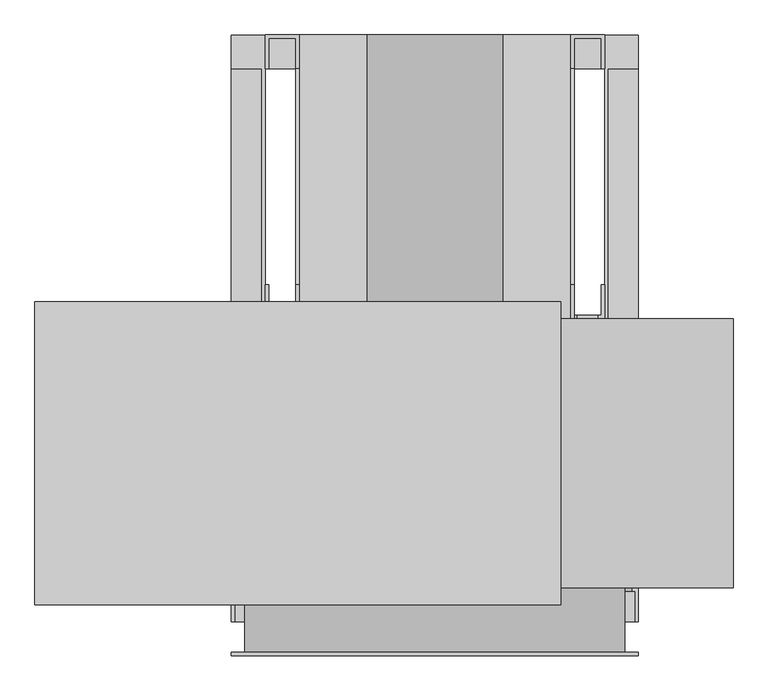
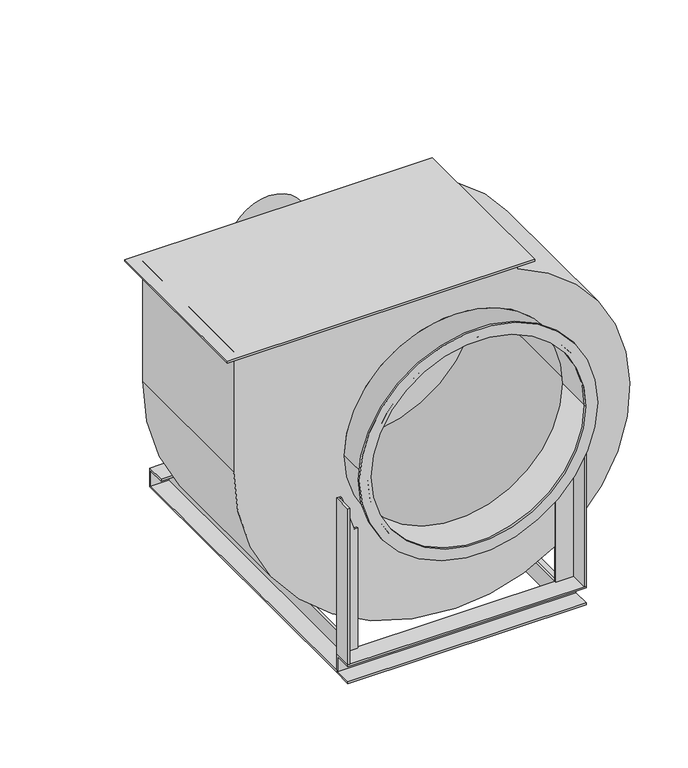
"""IFC4 building model written with IfcOpenShell, lengths in millimetres: proxy geometry, ВЕЗА_Вентилятор ВРАН : ВРАН6-056."""

import ifcopenshell
import ifcopenshell.guid

model = None  # the IFC model being written
_history = None  # IfcOwnerHistory: only IFC2X3 demands one
_inside = {}  # id of a spatial element -> (the spatial element, [elements in it])
_under = {}  # id of a project, library or spatial element -> (it, [spatial elements below it])
_declared = {}  # id of a project -> (the project, [libraries it declares])
_typed = {}  # id of a type object -> (the type object, [elements of that type])
_made_of = {}  # id of a material, layer set ... -> (it, [elements and type objects made of it])


def new_model(schema):
    """Start an empty IFC model of exactly this schema.

    Asked for "IFC4X3", IfcOpenShell would pick the latest addendum, in which some entities
    have other attributes; the version numbers below select the first issue.
    IFC2X3 requires an IfcOwnerHistory on every rooted entity: one is made here for all.
    """
    global model, _history
    if schema == "IFC4X3":
        model = ifcopenshell.file(schema_version=(4, 3, 0, 0))
    else:
        model = ifcopenshell.file(schema=schema)
    _inside.clear()
    _under.clear()
    _declared.clear()
    _typed.clear()
    _made_of.clear()
    _history = None
    if model.schema == "IFC2X3":
        org = make("IfcOrganization", Name="unknown")
        user = make(
            "IfcPersonAndOrganization",
            ThePerson=make("IfcPerson", FamilyName="unknown"),
            TheOrganization=org,
        )
        app = make(
            "IfcApplication",
            ApplicationDeveloper=org,
            Version="unknown",
            ApplicationFullName="unknown",
            ApplicationIdentifier="unknown",
        )
        _history = make(
            "IfcOwnerHistory",
            OwningUser=user,
            OwningApplication=app,
            ChangeAction="ADDED",
            CreationDate=0,
        )
    return model


def make(cls, **values):
    """One entity of the class cls with the attributes given. An attribute that is None is left unset."""
    return model.create_entity(
        cls, **{name: value for name, value in values.items() if value is not None}
    )


def rooted(cls, **values):
    """An entity with a GlobalId (a new one), such as an element, a storey or a relation."""
    return make(cls, GlobalId=ifcopenshell.guid.new(), OwnerHistory=_history, **values)


def si_unit(unit_type, name, prefix=None):
    """IfcSIUnit, for example si_unit("LENGTHUNIT", "METRE", prefix="MILLI")."""
    return make("IfcSIUnit", UnitType=unit_type, Prefix=prefix, Name=name)


def assignment(units):
    """IfcUnitAssignment: the units of a project."""
    return None if units is None else make("IfcUnitAssignment", Units=units)


def point(xyz):
    """IfcCartesianPoint."""
    return None if xyz is None else make("IfcCartesianPoint", Coordinates=xyz)


def direction(xyz):
    """IfcDirection."""
    return None if xyz is None else make("IfcDirection", DirectionRatios=xyz)


def frame(location, z_axis=None, x_axis=None):
    """IfcAxis2Placement3D, a coordinate frame: its origin and axes. An axis left out is left unset."""
    return make(
        "IfcAxis2Placement3D",
        Location=point(location),
        Axis=direction(z_axis),
        RefDirection=direction(x_axis),
    )


def frame_2d(location, x_axis=None):
    """IfcAxis2Placement2D, a coordinate frame in the plane: its origin and x axis."""
    return make(
        "IfcAxis2Placement2D", Location=point(location), RefDirection=direction(x_axis)
    )


def origin():
    """The frame at (0, 0, 0) with its axes left unset."""
    return frame((0.0, 0.0, 0.0))


def place(relative_to, where):
    """IfcLocalPlacement: puts the frame where relative to a parent placement (None: the world)."""
    return make(
        "IfcLocalPlacement", PlacementRelTo=relative_to, RelativePlacement=where
    )


def context(
    kind, dimensions, precision=None, world=None, true_north=None, identifier=None
):
    """IfcGeometricRepresentationContext, for example the 3D "Model" context."""
    return make(
        "IfcGeometricRepresentationContext",
        ContextIdentifier=identifier,
        ContextType=kind,
        CoordinateSpaceDimension=dimensions,
        Precision=precision,
        WorldCoordinateSystem=world,
        TrueNorth=true_north,
    )


def project(units=None, contexts=None):
    """IfcProject with its units and contexts."""
    return rooted(
        "IfcProject",
        Name="project",
        RepresentationContexts=contexts,
        UnitsInContext=assignment(units),
    )


def spatial(cls, under=None, at=None, **own):
    """A site, building, storey or space (cls), placed at a placement, below another one or the project."""
    s = rooted(cls, ObjectPlacement=at, **own)
    if under is not None:
        _under.setdefault(under.id(), (under, []))[1].append(s)
    return s


def polyline(points):
    """IfcPolyline through the points."""
    return make("IfcPolyline", Points=[point(p) for p in points])


def circle_curve(where, radius):
    """IfcCircle in the frame where."""
    return make("IfcCircle", Position=where, Radius=radius)


def trimmed(basis, trim1, trim2, sense, master):
    """IfcTrimmedCurve: the piece of a basis curve between two trims."""
    return make(
        "IfcTrimmedCurve",
        BasisCurve=basis,
        Trim1=trim1,
        Trim2=trim2,
        SenseAgreement=sense,
        MasterRepresentation=master,
    )


def segment(curve, same_sense, transition):
    """IfcCompositeCurveSegment."""
    return make(
        "IfcCompositeCurveSegment",
        Transition=transition,
        SameSense=same_sense,
        ParentCurve=curve,
    )


def composite_curve(segments, self_intersect=None):
    """IfcCompositeCurve: segments joined end to end."""
    return make("IfcCompositeCurve", Segments=segments, SelfIntersect=self_intersect)


def outline(outer, holes=None, kind="AREA"):
    """IfcArbitraryClosedProfileDef: a profile drawn as a closed curve; with holes, ...WithVoids."""
    if holes is None:
        return make("IfcArbitraryClosedProfileDef", ProfileType=kind, OuterCurve=outer)
    return make(
        "IfcArbitraryProfileDefWithVoids",
        ProfileType=kind,
        OuterCurve=outer,
        InnerCurves=holes,
    )


def extrude(swept, where, along, depth):
    """IfcExtrudedAreaSolid: the profile swept, set in the frame where, extruded along a direction by depth."""
    return make(
        "IfcExtrudedAreaSolid",
        SweptArea=swept,
        Position=where,
        ExtrudedDirection=direction(along),
        Depth=depth,
    )


def faces_of(points, faces, orient=None, outer=None):
    """IfcFace entities. A face is a list of loops; a loop is a list of indices into points, from 0.

    orient and outer hold one flag for each loop. By default every Orientation is true, the
    first loop of a face is its IfcFaceOuterBound and the others are IfcFaceBound.
    """
    made = []
    for i, loops in enumerate(faces):
        bounds = []
        for j, loop in enumerate(loops):
            is_outer = j == 0 if outer is None else outer[i][j]
            bounds.append(
                make(
                    "IfcFaceOuterBound" if is_outer else "IfcFaceBound",
                    Bound=make("IfcPolyLoop", Polygon=[points[k] for k in loop]),
                    Orientation=True if orient is None else orient[i][j],
                )
            )
        made.append(make("IfcFace", Bounds=bounds))
    return made


def faceted_brep(points, faces, orient=None, outer=None, voids=None):
    """IfcFacetedBrep: a solid bounded by flat faces; with voids (closed shells), ...WithVoids."""
    shared = [point(p) for p in points]
    hull = make("IfcClosedShell", CfsFaces=faces_of(shared, faces, orient, outer))
    if voids is None:
        return make("IfcFacetedBrep", Outer=hull)
    return make(
        "IfcFacetedBrepWithVoids",
        Outer=hull,
        Voids=[
            make(cls, CfsFaces=faces_of(shared, fs, o, b)) for cls, fs, o, b in voids
        ],
    )


def shape(context_of_items, identifier, shape_type, items):
    """IfcShapeRepresentation: the items that make up one representation, for example the "Body"."""
    return make(
        "IfcShapeRepresentation",
        ContextOfItems=context_of_items,
        RepresentationIdentifier=identifier,
        RepresentationType=shape_type,
        Items=items,
    )


def source(mapping_origin, context_of_items, identifier, shape_type, items):
    """IfcRepresentationMap: a shape defined once, which mapped items show again and again."""
    return make(
        "IfcRepresentationMap",
        MappingOrigin=mapping_origin,
        MappedRepresentation=shape(context_of_items, identifier, shape_type, items),
    )


def transform(
    local_origin,
    x_axis=None,
    y_axis=None,
    z_axis=None,
    scale=None,
    scale2=None,
    scale3=None,
    uniform=True,
):
    """IfcCartesianTransformationOperator3D, or its non-uniform kind. x_axis, y_axis, z_axis: its Axis1, 2, 3."""
    if uniform:
        return make(
            "IfcCartesianTransformationOperator3D",
            Axis1=direction(x_axis),
            Axis2=direction(y_axis),
            LocalOrigin=point(local_origin),
            Scale=scale,
            Axis3=direction(z_axis),
        )
    return make(
        "IfcCartesianTransformationOperator3DnonUniform",
        Axis1=direction(x_axis),
        Axis2=direction(y_axis),
        LocalOrigin=point(local_origin),
        Scale=scale,
        Axis3=direction(z_axis),
        Scale2=scale2,
        Scale3=scale3,
    )


def mapped(mapping_source, mapping_target):
    """IfcMappedItem: shows the shape of a source again, moved by a transform."""
    return make(
        "IfcMappedItem", MappingSource=mapping_source, MappingTarget=mapping_target
    )


def made_of(thing, what):
    """Note that an element or type object is made of a material, layer set ...; save() writes the relation."""
    if what is not None:
        _made_of.setdefault(what.id(), (what, []))[1].append(thing)
    return thing


def element(
    cls,
    number,
    at=None,
    inside=None,
    cuts=None,
    type_object=None,
    material=None,
    context=None,
    identifier="Body",
    shape_type=None,
    held_by="IfcProductDefinitionShape",
    body=None,
    shapes=None,
    **own,
):
    """One element of the class cls, such as IfcWall. Its Tag is "e" and its number.

    at: its placement. inside: the storey or other place that contains it. cuts: it is an
    opening in that element (IfcRelVoidsElement). A single representation is given by context,
    identifier, shape_type and body (its items); several are given by shapes. held_by: the class
    of the entity that holds the representations. save() writes the other relations.
    """
    e = rooted(cls, Tag="e%d" % number, ObjectPlacement=at, **own)
    if body is not None:
        shapes = [shape(context, identifier, shape_type, body)]
    if shapes is not None:
        e.Representation = make(held_by, Representations=shapes)
    if inside is not None:
        _inside.setdefault(inside.id(), (inside, []))[1].append(e)
    if cuts is not None:
        rooted(
            "IfcRelVoidsElement", RelatingBuildingElement=cuts, RelatedOpeningElement=e
        )
    if type_object is not None:
        _typed.setdefault(type_object.id(), (type_object, []))[1].append(e)
    return made_of(e, material)


def aggregate(whole, parts):
    """IfcRelAggregates: a whole, such as a stair, and the parts it consists of."""
    return rooted("IfcRelAggregates", RelatingObject=whole, RelatedObjects=parts)


def save(model, path):
    """Write the relations noted so far, then the file.

    IfcRelAggregates (storeys below a building ...), IfcRelContainedInSpatialStructure (elements
    in a storey), IfcRelDefinesByType, IfcRelAssociatesMaterial and IfcRelDeclares: one each for
    every whole, place, type object, material and project.
    """
    for whole, parts in _under.values():
        aggregate(whole, parts)
    for where, things in _inside.values():
        rooted(
            "IfcRelContainedInSpatialStructure",
            RelatedElements=things,
            RelatingStructure=where,
        )
    for kind, things in _typed.values():
        rooted("IfcRelDefinesByType", RelatedObjects=things, RelatingType=kind)
    for what, things in _made_of.values():
        rooted("IfcRelAssociatesMaterial", RelatedObjects=things, RelatingMaterial=what)
    for by, libraries in _declared.values():
        rooted("IfcRelDeclares", RelatingContext=by, RelatedDefinitions=libraries)
    model.write(path)


def mechanical_equipment_89e30f27(model_context):
    return source(origin(), model_context, "Body", "SolidModel", [
        extrude(outline(polyline([(185.5, 223.5), (185.5, -223.5), (-589.5, -223.5), (-589.5, 223.5), (185.5, 223.5)])), frame((0.0, 0.0, 940.0), z_axis=(0.0, 0.0, 1.0), x_axis=(1.0, 0.0, 0.0)), (0.0, 0.0, 1.0), 5.0),
        extrude(outline(composite_curve([segment(trimmed(circle_curve(frame_2d((625.0, 0.5002234)), 560.0002234), [point((625.0, -559.5))], [point((65.0, 0.0))], False, "CARTESIAN"), True, "CONTINUOUS"), segment(trimmed(circle_curve(frame_2d((504.1653304, 0.3189338)), 439.1654462), [point((65.0, 0.0))], [point((915.0, 155.5))], False, "CARTESIAN"), True, "CONTINUOUS"), segment(polyline([(915.0, 155.5), (945.0, 155.5), (945.0, -559.5), (625.0, -559.5)]), True, "CONTINUOUS")], self_intersect=False), holes=[composite_curve([segment(trimmed(circle_curve(frame_2d((570.0, 0.0)), 280.0), [point((570.0, -280.0))], [point((570.0, 280.0))], True, "CARTESIAN"), True, "CONTINUOUS"), segment(trimmed(circle_curve(frame_2d((570.0, 0.0)), 280.0), [point((570.0, 280.0))], [point((570.0, -280.0))], True, "CARTESIAN"), True, "CONTINUOUS")], self_intersect=False)]), frame((0.0, -198.5, 0.0), z_axis=(0.0, 1.0, 0.0), x_axis=(0.0, 0.0, 1.0)), (0.0, 0.0, 1.0), 397.0),
        faceted_brep([(-300.0, 611.5, 5.0), (-300.0, 611.5, 45.0), (-300.0, 566.5, 45.0), (-300.0, 566.5, 50.0), (-300.0, 616.5, 50.0), (-300.0, 616.5, 0.0), (-300.0, -198.5, 0.0), (-300.0, -198.5, 5.0), (300.0, 616.5, 50.0), (300.0, 566.5, 50.0), (300.0, 566.5, 45.0), (300.0, 611.5, 45.0), (300.0, 611.5, 5.0), (300.0, -198.5, 5.0), (300.0, -198.5, 0.0), (300.0, 616.5, 0.0), (250.0, -198.5, 0.0), (250.0, 566.5, 0.0), (-250.0, 566.5, 0.0), (-250.0, -198.5, 0.0), (-255.0, 566.5, 45.0), (-255.0, 566.5, 50.0), (255.0, 566.5, 50.0), (255.0, 566.5, 45.0), (-200.0, 566.5, 470.0), (-205.0, 566.5, 470.0), (-205.0, 566.5, 50.0), (-245.0, 566.5, 50.0), (-245.0, 566.5, 470.0), (-250.0, 566.5, 470.0), (-250.0, 566.5, 50.0), (250.0, 566.5, 50.0), (250.0, 566.5, 470.0), (245.0, 566.5, 470.0), (245.0, 566.5, 50.0), (205.0, 566.5, 50.0), (205.0, 566.5, 470.0), (200.0, 566.5, 470.0), (200.0, 566.5, 50.0), (-200.0, 566.5, 50.0), (205.0, 566.5, 5.0), (205.0, 566.5, 45.0), (245.0, 566.5, 45.0), (245.0, 566.5, 5.0), (-245.0, 566.5, 5.0), (-245.0, 566.5, 45.0), (-205.0, 566.5, 45.0), (-205.0, 566.5, 5.0), (-200.0, 566.5, 5.0), (-200.0, 566.5, 45.0), (200.0, 566.5, 45.0), (200.0, 566.5, 5.0), (245.0, 611.5, 5.0), (205.0, 611.5, 5.0), (-205.0, 611.5, 5.0), (-245.0, 611.5, 5.0), (200.0, 611.5, 5.0), (-200.0, 611.5, 5.0), (255.0, -198.5, 5.0), (255.0, 611.5, 5.0), (-255.0, -198.5, 5.0), (-255.0, 611.5, 5.0), (-255.0, 611.5, 45.0), (255.0, 611.5, 45.0), (245.0, 611.5, 45.0), (205.0, 611.5, 45.0), (-205.0, 611.5, 45.0), (-245.0, 611.5, 45.0), (200.0, 611.5, 45.0), (-200.0, 611.5, 45.0), (-255.0, -198.5, 50.0), (-250.0, -198.5, 50.0), (-250.0, 616.5, 50.0), (250.0, 616.5, 50.0), (250.0, -198.5, 50.0), (255.0, -198.5, 50.0), (-205.0, 611.5, 50.0), (-245.0, 611.5, 50.0), (245.0, 611.5, 50.0), (205.0, 611.5, 50.0), (200.0, 616.5, 50.0), (-200.0, 616.5, 50.0), (-250.0, 616.5, 470.0), (-200.0, 616.5, 470.0), (200.0, 616.5, 470.0), (250.0, 616.5, 470.0), (-245.0, 611.5, 470.0), (-205.0, 611.5, 470.0), (205.0, 611.5, 470.0), (245.0, 611.5, 470.0)], [[[0, 1, 2, 3, 4, 5, 6, 7]], [[8, 9, 10, 11, 12, 13, 14, 15]], [[14, 16, 17, 18, 19, 6, 5, 15]], [[3, 2, 20, 21]], [[10, 9, 22, 23]], [[24, 25, 26, 27, 28, 29, 30, 18, 17, 31, 32, 33, 34, 35, 36, 37, 38, 39], [40, 41, 42, 43], [44, 45, 46, 47], [48, 49, 50, 51]], [[40, 43, 52, 53]], [[44, 47, 54, 55]], [[48, 51, 56, 57]], [[58, 13, 12, 59]], [[7, 60, 61, 0]], [[1, 0, 61, 62]], [[12, 11, 63, 59]], [[53, 52, 64, 65]], [[55, 54, 66, 67]], [[57, 56, 68, 69]], [[2, 1, 62, 20]], [[11, 10, 23, 63]], [[65, 64, 42, 41]], [[67, 66, 46, 45]], [[69, 68, 50, 49]], [[4, 3, 21, 70, 71, 30, 72]], [[9, 8, 73, 31, 74, 75, 22]], [[27, 26, 76, 77]], [[35, 34, 78, 79]], [[39, 38, 80, 81]], [[8, 15, 5, 4, 72, 82, 83, 81, 80, 84, 85, 73]], [[75, 74, 16, 14, 13, 58]], [[75, 58, 59, 63, 23, 22]], [[16, 74, 31, 17]], [[70, 60, 7, 6, 19, 71]], [[60, 70, 21, 20, 62, 61]], [[71, 19, 18, 30]], [[83, 82, 29, 28, 86, 87, 25, 24]], [[84, 37, 36, 88, 89, 33, 32, 85]], [[89, 88, 79, 78]], [[43, 42, 64, 52]], [[33, 89, 78, 34]], [[85, 32, 31, 73]], [[51, 50, 68, 56]], [[37, 84, 80, 38]], [[41, 40, 53, 65]], [[88, 36, 35, 79]], [[29, 82, 72, 30]], [[45, 44, 55, 67]], [[86, 28, 27, 77]], [[87, 86, 77, 76]], [[47, 46, 66, 54]], [[25, 87, 76, 26]], [[49, 48, 57, 69]], [[83, 24, 39, 81]]]),
        extrude(outline(polyline([(566.5, 0.0), (198.5, 0.0), (198.5, 770.0), (248.5420316, 770.0), (566.5, 510.0420316), (566.5, 0.0)]), holes=[polyline([(248.5, 495.0), (486.5, 495.0), (486.5, 501.5949723), (273.4504813, 670.0), (248.5, 670.0), (248.5, 495.0)])]), frame((-205.0, 0.0, 0.0), z_axis=(1.0, 0.0, 0.0), x_axis=(0.0, 1.0, 0.0)), (0.0, 0.0, 1.0), 5.0),
        faceted_brep([(250.0, -198.5, 50.0), (300.0, -198.5, 50.0), (300.0, -248.5, 50.0), (295.0, -248.5, 50.0), (295.0, -203.5, 50.0), (250.0, -203.5, 50.0), (250.0, -198.5, 370.0), (258.2904546, -198.5, 370.0), (289.966699, -198.5, 465.0), (300.0, -198.5, 465.0), (300.0, -248.5, 465.0), (295.0, -248.5, 465.0), (295.0, -203.5, 465.0), (289.966699, -203.5, 465.0), (258.2904546, -203.5, 370.0), (250.0, -203.5, 370.0)], [[[0, 1, 2, 3, 4, 5]], [[1, 0, 6, 7, 8, 9]], [[2, 1, 9, 10]], [[3, 2, 10, 11]], [[4, 3, 11, 12]], [[5, 4, 12, 13, 14, 15]], [[0, 5, 15, 6]], [[14, 7, 6, 15]], [[7, 14, 13, 8]], [[8, 13, 12, 11, 10, 9]]]),
        faceted_brep([(-250.0, -198.5, 50.0), (-250.0, -203.5, 50.0), (-295.0, -203.5, 50.0), (-295.0, -248.5, 50.0), (-300.0, -248.5, 50.0), (-300.0, -198.5, 50.0), (-250.0, -198.5, 370.0), (-250.0, -203.5, 370.0), (-258.2904546, -203.5, 370.0), (-289.966699, -203.5, 465.0), (-295.0, -203.5, 465.0), (-295.0, -248.5, 465.0), (-300.0, -248.5, 465.0), (-300.0, -198.5, 465.0), (-289.966699, -198.5, 465.0), (-258.2904546, -198.5, 370.0)], [[[0, 1, 2, 3, 4, 5]], [[1, 0, 6, 7]], [[2, 1, 7, 8, 9, 10]], [[3, 2, 10, 11]], [[4, 3, 11, 12]], [[5, 4, 12, 13]], [[0, 5, 13, 14, 15, 6]], [[9, 14, 13, 12, 11, 10]], [[14, 9, 8, 15]], [[15, 8, 7, 6]]]),
        extrude(outline(polyline([(566.5, 0.0), (198.5, 0.0), (198.5, 770.0), (248.5420316, 770.0), (566.5, 510.0420316), (566.5, 0.0)]), holes=[polyline([(248.5, 495.0), (486.5, 495.0), (486.5, 501.5949723), (273.4504813, 670.0), (248.5, 670.0), (248.5, 495.0)])]), frame((200.0, 0.0, 0.0), z_axis=(1.0, 0.0, 0.0), x_axis=(0.0, 1.0, 0.0)), (0.0, 0.0, 1.0), 5.0),
        faceted_brep([(200.0, 198.5, 0.0), (200.0, 203.5, 0.0), (245.0, 203.5, 0.0), (245.0, 248.5, 0.0), (250.0, 248.5, 0.0), (250.0, 198.5, 0.0), (250.0, 198.5, 680.0), (240.0, 198.5, 680.0), (208.75409, 198.5, 763.6095143), (200.0, 198.5, 763.6095143), (250.0, 248.5, 680.0), (245.0, 248.5, 680.0), (245.0, 203.5, 680.0), (200.0, 203.5, 763.6095143), (208.75409, 203.5, 763.6095143), (240.0, 203.5, 680.0)], [[[0, 1, 2, 3, 4, 5]], [[0, 5, 6, 7, 8, 9]], [[5, 4, 10, 6]], [[4, 3, 11, 10]], [[3, 2, 12, 11]], [[2, 1, 13, 14, 15, 12]], [[1, 0, 9, 13]], [[8, 14, 13, 9]], [[14, 8, 7, 15]], [[15, 7, 6, 10, 11, 12]]]),
        faceted_brep([(-200.0, 198.5, 0.0), (-250.0, 198.5, 0.0), (-250.0, 248.5, 0.0), (-245.0, 248.5, 0.0), (-245.0, 203.5, 0.0), (-200.0, 203.5, 0.0), (-200.0, 203.5, 763.6095143), (-200.0, 198.5, 763.6095143), (-245.0, 203.5, 680.0), (-240.0, 203.5, 680.0), (-208.75409, 203.5, 763.6095143), (-245.0, 248.5, 680.0), (-250.0, 248.5, 680.0), (-250.0, 198.5, 680.0), (-208.75409, 198.5, 763.6095143), (-240.0, 198.5, 680.0)], [[[0, 1, 2, 3, 4, 5]], [[0, 5, 6, 7]], [[5, 4, 8, 9, 10, 6]], [[4, 3, 11, 8]], [[3, 2, 12, 11]], [[2, 1, 13, 12]], [[1, 0, 7, 14, 15, 13]], [[15, 9, 8, 11, 12, 13]], [[9, 15, 14, 10]], [[10, 14, 7, 6]]]),
        extrude(outline(polyline([(-198.5, 50.0), (-198.5, 0.0), (-248.5, 0.0), (-248.5, 5.0), (-203.5, 5.0), (-203.5, 45.0), (-248.5, 45.0), (-248.5, 50.0), (-198.5, 50.0)])), frame((-300.0, 0.0, 0.0), z_axis=(1.0, 0.0, 0.0), x_axis=(0.0, 1.0, 0.0)), (0.0, 0.0, 1.0), 600.0),
        extrude(outline(composite_curve([segment(trimmed(circle_curve(frame_2d((570.0, 0.0)), 280.0), [point((570.0, -280.0))], [point((570.0, 280.0))], False, "CARTESIAN"), True, "CONTINUOUS"), segment(trimmed(circle_curve(frame_2d((570.0, 0.0)), 280.0), [point((570.0, 280.0))], [point((570.0, -280.0))], False, "CARTESIAN"), True, "CONTINUOUS")], self_intersect=False)), frame((0.0, 193.5, 0.0), z_axis=(0.0, 1.0, 0.0), x_axis=(0.0, 0.0, 1.0)), (0.0, 0.0, 1.0), 5.0),
        extrude(outline(composite_curve([segment(trimmed(circle_curve(frame_2d((570.0, 0.0)), 300.0), [point((570.0, -300.0))], [point((570.0, 300.0))], False, "CARTESIAN"), True, "CONTINUOUS"), segment(trimmed(circle_curve(frame_2d((570.0, 0.0)), 300.0), [point((570.0, 300.0))], [point((570.0, -300.0))], False, "CARTESIAN"), True, "CONTINUOUS")], self_intersect=False), holes=[composite_curve([segment(trimmed(circle_curve(frame_2d((570.0, 0.0)), 270.0), [point((570.0, -270.0))], [point((570.0, 270.0))], True, "CARTESIAN"), True, "CONTINUOUS"), segment(trimmed(circle_curve(frame_2d((570.0, 0.0)), 270.0), [point((570.0, 270.0))], [point((570.0, -270.0))], True, "CARTESIAN"), True, "CONTINUOUS")], self_intersect=False)]), frame((0.0, -298.5, 0.0), z_axis=(0.0, 1.0, 0.0), x_axis=(0.0, 0.0, 1.0)), (0.0, 0.0, 1.0), 5.0),
        extrude(outline(polyline([(200.0, 616.5), (200.0, 198.5), (-200.0, 198.5), (-200.0, 616.5), (200.0, 616.5)])), frame((0.0, 0.0, 420.0), z_axis=(0.0, 0.0, 1.0), x_axis=(1.0, 0.0, 0.0)), (0.0, 0.0, 1.0), 50.0),
        extrude(outline(composite_curve([segment(trimmed(circle_curve(frame_2d((570.0, 0.0)), 100.0), [point((570.0, 100.0))], [point((570.0, -100.0))], False, "CARTESIAN"), True, "CONTINUOUS"), segment(trimmed(circle_curve(frame_2d((570.0, 0.0)), 100.0), [point((570.0, -100.0))], [point((570.0, 100.0))], False, "CARTESIAN"), True, "CONTINUOUS")], self_intersect=False)), frame((0.0, 198.5, 0.0), z_axis=(0.0, 1.0, 0.0), x_axis=(0.0, 0.0, 1.0)), (0.0, 0.0, 1.0), 418.0),
        extrude(outline(composite_curve([segment(trimmed(circle_curve(frame_2d((570.0, 0.0)), 280.0), [point((570.0, 280.0))], [point((570.0, -280.0))], False, "CARTESIAN"), True, "CONTINUOUS"), segment(trimmed(circle_curve(frame_2d((570.0, 0.0)), 280.0), [point((570.0, -280.0))], [point((570.0, 280.0))], False, "CARTESIAN"), True, "CONTINUOUS")], self_intersect=False), holes=[composite_curve([segment(trimmed(circle_curve(frame_2d((570.0, 0.0)), 270.0), [point((570.0, 270.0))], [point((570.0, -270.0))], True, "CARTESIAN"), True, "CONTINUOUS"), segment(trimmed(circle_curve(frame_2d((570.0, 0.0)), 270.0), [point((570.0, -270.0))], [point((570.0, 270.0))], True, "CARTESIAN"), True, "CONTINUOUS")], self_intersect=False)]), frame((0.0, -298.5, 0.0), z_axis=(0.0, 1.0, 0.0), x_axis=(0.0, 0.0, 1.0)), (0.0, 0.0, 1.0), 100.0),
    ])


if __name__ == "__main__":
    model = new_model("IFC4")
    model_context = context("Model", 3, world=origin())
    ifc_project = project(units=[si_unit("LENGTHUNIT", "METRE", prefix="MILLI")], contexts=[model_context])
    site = spatial("IfcSite", under=ifc_project)
    building = spatial("IfcBuilding", under=site)
    placement = place(None, origin())
    mechanical_equipment_shape = mechanical_equipment_89e30f27(model_context)
    element("IfcBuildingElementProxy", 1, Name="ВЕЗА_Вентилятор ВРАН : ВРАН6-056", ObjectType="ВЕЗА_Вентилятор ВРАН : ВРАН6-056", at=placement, inside=building, context=model_context, shape_type="MappedRepresentation", body=[
        mapped(mechanical_equipment_shape, transform((0.0, 0.0, 0.0), x_axis=(1.0, 0.0, 0.0), y_axis=(0.0, 1.0, 0.0), z_axis=(0.0, 0.0, 1.0))),
    ])
    save(model, "model.ifc")

# Revit data of these elements
# Type "ВЕЗА_Вентилятор ВРАН : ВРАН6-056"
#   УголВысота = "ВРАН_Угол_Высота"
#   ADSK_Этаж [instance default] = ""
#   ADSK_Примечание [instance default] = ""
#   ADSK_Позиция = "9"
#   ADSK_Обозначение = ""
#   ADSK_Наименование = "Вентилятор радиальный ВРАН6; типоразмер 056; режим работы Т80; исполнение взрывозащищенное коррозионностойкое; номинальная мощность Nном=2,2кВт, число полюсов 4; климатическое исполнение УХЛ2; конструктивное исполнение 1; положение корпуса ПО; без ТШК"
#   О_Назначение [instance default] = ""
#   ADSK_Марка = "ВРАН6-056-Т80-ВК1-00220/4-УХЛ2-1-ПО-О ТУ 4861-104-40149153-2007"
#   ADSK_Комплект [instance default] = ""
#   ADSK_Код изделия = "4039929"
#   ADSK_Зона [instance default] = ""
#   ADSK_Единица измерения = "компл."
#   И_НаименованиеФитинга = ""
#   И_НаименованиеСистемы [instance default] = ""
#   И_КодОборудования = "ВРАН6-056-П0-0"
#   ADSK_Завод-изготовитель = "ООО \"Веза\", Россия, Москва, ИНН 505001001, info@veza.ru"
#   Габариты = "vran_du"
#   ШиринаСтойкиОкна2 = 100 mm
#   ШиринаСтойкиОкна1 = 130 mm
#   ШиринаСтойкиДвигателя = 50 mm
#   Уголок = 50 mm
#   УголНаклона [instance default] = 0°
#   Угол [instance default] = 0°
#   Столик = -50 mm
#   Расход [instance default] = 0 m³/h
#   ADSK_Масса = 100
#   ADSK_Количество = 1
#   ADSK_Номинальная мощность [instance default] = 0 W
#   РадиусДвигателя = 100 mm
#   НомерВентилятора = 5.6 mm
#   ВысотаПлощадкиДвигателя [instance default] = 470 mm
#   ВерхОпор = 200 mm
#   R3 = 300 mm
#   R2 = 270 mm
#   Lmax = 865 mm
#   h [instance default] = 570 mm
#   R = 280 mm
#   L2 = 202 mm
#   H = 945 mm
#   D = 560 mm
#   C = 550 mm
#   B_корпуса = 1020 mm
#   B = 720 mm
#   A = 397 mm
#   Швеллер = yes
#   Default Elevation = 0
#   Type Comments = ""
